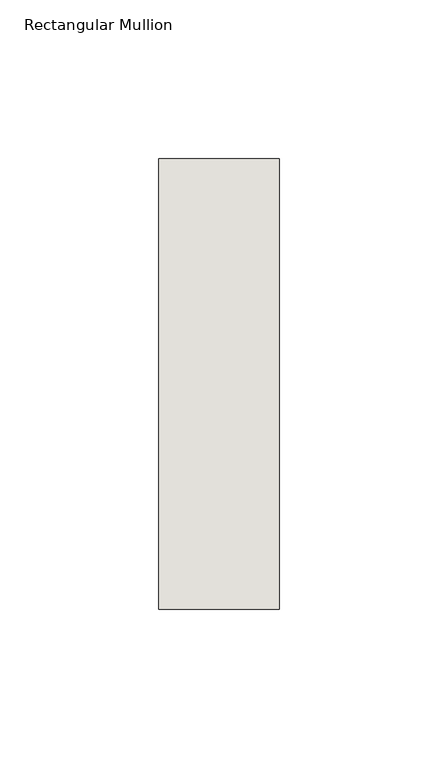
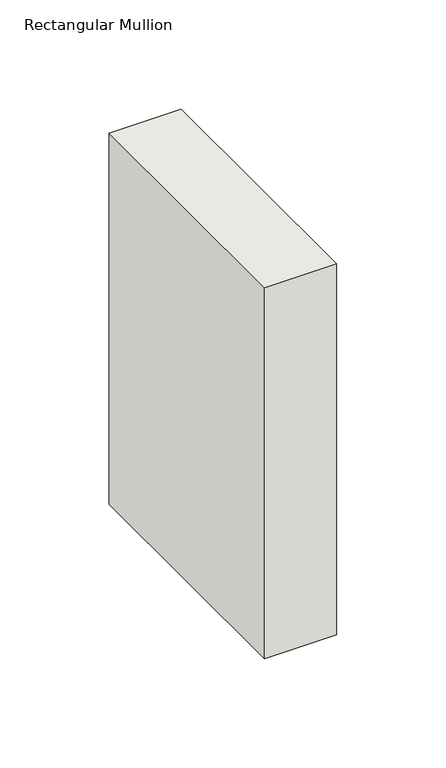
"""IFC4 building model written with IfcOpenShell, lengths in millimetres: wall geometry, Rectangular Mullion : NLRS_21_CWM_hsb-regel 38x142_gen_rsf."""

from ifc_helpers import new_model, si_unit, frame, origin, place, context, project, spatial, polyline, outline, extrude, source, transform, mapped, element, save


def rectangular_mullion_345d7182(model_context):
    return source(origin(), model_context, "Body", "SweptSolid", [
        extrude(outline(polyline([(-38.0, -71.0), (-38.0, 71.0), (0.0, 71.0), (0.0, -71.0), (-38.0, -71.0)])), frame((0.0, 0.0, -207.0000003), z_axis=(0.0, 0.0, 1.0), x_axis=(1.0, 0.0, 0.0)), (0.0, 0.0, 1.0), 207.0000003),
    ])


if __name__ == "__main__":
    model = new_model("IFC4")
    model_context = context("Model", 3, world=origin())
    ifc_project = project(units=[si_unit("LENGTHUNIT", "METRE", prefix="MILLI")], contexts=[model_context])
    site = spatial("IfcSite", under=ifc_project)
    building = spatial("IfcBuilding", under=site)
    placement = place(None, origin())
    rectangular_mullion_shape = rectangular_mullion_345d7182(model_context)
    element("IfcWall", 1, ObjectType="Rectangular Mullion : NLRS_21_CWM_hsb-regel 38x142_gen_rsf", at=placement, inside=building, context=model_context, shape_type="MappedRepresentation", body=[
        mapped(rectangular_mullion_shape, transform((0.0, 0.0, 0.0), x_axis=(1.0, 0.0, 0.0), y_axis=(0.0, 1.0, 0.0), z_axis=(0.0, 0.0, 1.0))),
    ])
    save(model, "model.ifc")

# Revit data of these elements
# Type "Rectangular Mullion : NLRS_21_CWM_hsb-regel 38x142_gen_rsf"
#   Type IfcGUID = "07M7mRoiH1CR8m_RSKIwpF"
#   Assembly Code = "21.10"
#   IfcExportAs = "IfcWall"
#   built-in parameter 1007322 = 0.465879 (stored number, unit not read)
#   built-in parameter 1007321 = 0.062336 (stored number, unit not read)
#   built-in parameter 1007320 = 0.062336 (stored number, unit not read)
# Element 1 (IfcWall, "Rectangular Mullion : NLRS_21_CWM_hsb-regel 38x142_gen_rsf")
#   Materials on its faces: "NLRS_i2_hout naaldhout vuren_gen_rsf"
# Materials
#   "NLRS_i2_hout naaldhout vuren_gen_rsf": class "I - Hout", colour RGB 234 199 147, transparency 0, Keynote = "i2", Manufacturer = "Revit Standards Foundation", URL = "www.revitstandards.org", Description = "hout vuren", Cost = 0
